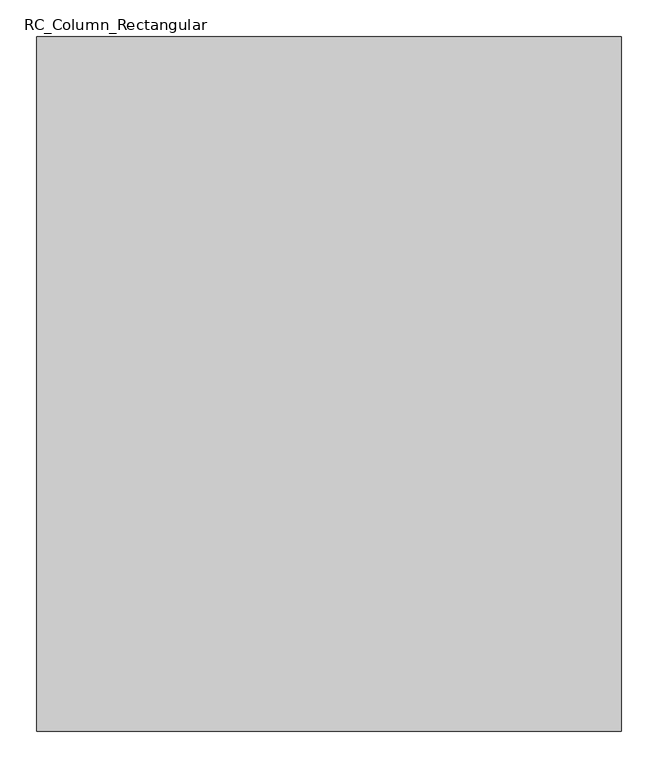
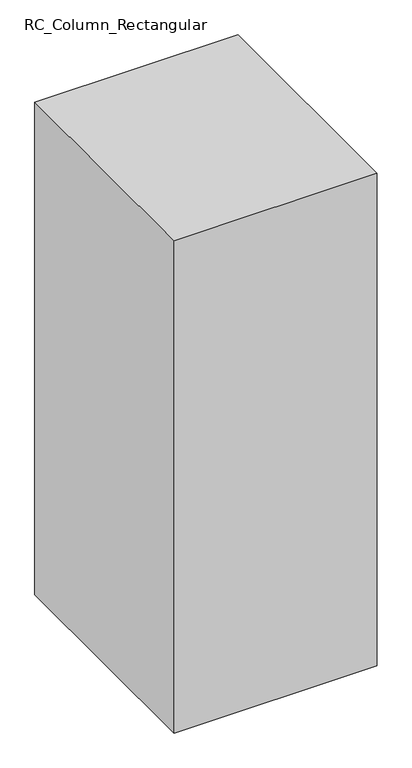
"""IFC4 building model written with IfcOpenShell, lengths in millimetres: column geometry, RC_Column_Rectangular : H_SC_AR_S15_UG PED_W800xL950_Bit_PD1."""

import ifcopenshell
import ifcopenshell.guid

model = None  # the IFC model being written
_history = None  # IfcOwnerHistory: only IFC2X3 demands one
_inside = {}  # id of a spatial element -> (the spatial element, [elements in it])
_under = {}  # id of a project, library or spatial element -> (it, [spatial elements below it])
_declared = {}  # id of a project -> (the project, [libraries it declares])
_typed = {}  # id of a type object -> (the type object, [elements of that type])
_made_of = {}  # id of a material, layer set ... -> (it, [elements and type objects made of it])


def new_model(schema):
    """Start an empty IFC model of exactly this schema.

    Asked for "IFC4X3", IfcOpenShell would pick the latest addendum, in which some entities
    have other attributes; the version numbers below select the first issue.
    IFC2X3 requires an IfcOwnerHistory on every rooted entity: one is made here for all.
    """
    global model, _history
    if schema == "IFC4X3":
        model = ifcopenshell.file(schema_version=(4, 3, 0, 0))
    else:
        model = ifcopenshell.file(schema=schema)
    _inside.clear()
    _under.clear()
    _declared.clear()
    _typed.clear()
    _made_of.clear()
    _history = None
    if model.schema == "IFC2X3":
        org = make("IfcOrganization", Name="unknown")
        user = make(
            "IfcPersonAndOrganization",
            ThePerson=make("IfcPerson", FamilyName="unknown"),
            TheOrganization=org,
        )
        app = make(
            "IfcApplication",
            ApplicationDeveloper=org,
            Version="unknown",
            ApplicationFullName="unknown",
            ApplicationIdentifier="unknown",
        )
        _history = make(
            "IfcOwnerHistory",
            OwningUser=user,
            OwningApplication=app,
            ChangeAction="ADDED",
            CreationDate=0,
        )
    return model


def make(cls, **values):
    """One entity of the class cls with the attributes given. An attribute that is None is left unset."""
    return model.create_entity(
        cls, **{name: value for name, value in values.items() if value is not None}
    )


def rooted(cls, **values):
    """An entity with a GlobalId (a new one), such as an element, a storey or a relation."""
    return make(cls, GlobalId=ifcopenshell.guid.new(), OwnerHistory=_history, **values)


def si_unit(unit_type, name, prefix=None):
    """IfcSIUnit, for example si_unit("LENGTHUNIT", "METRE", prefix="MILLI")."""
    return make("IfcSIUnit", UnitType=unit_type, Prefix=prefix, Name=name)


def assignment(units):
    """IfcUnitAssignment: the units of a project."""
    return None if units is None else make("IfcUnitAssignment", Units=units)


def point(xyz):
    """IfcCartesianPoint."""
    return None if xyz is None else make("IfcCartesianPoint", Coordinates=xyz)


def direction(xyz):
    """IfcDirection."""
    return None if xyz is None else make("IfcDirection", DirectionRatios=xyz)


def frame(location, z_axis=None, x_axis=None):
    """IfcAxis2Placement3D, a coordinate frame: its origin and axes. An axis left out is left unset."""
    return make(
        "IfcAxis2Placement3D",
        Location=point(location),
        Axis=direction(z_axis),
        RefDirection=direction(x_axis),
    )


def origin():
    """The frame at (0, 0, 0) with its axes left unset."""
    return frame((0.0, 0.0, 0.0))


def place(relative_to, where):
    """IfcLocalPlacement: puts the frame where relative to a parent placement (None: the world)."""
    return make(
        "IfcLocalPlacement", PlacementRelTo=relative_to, RelativePlacement=where
    )


def context(
    kind, dimensions, precision=None, world=None, true_north=None, identifier=None
):
    """IfcGeometricRepresentationContext, for example the 3D "Model" context."""
    return make(
        "IfcGeometricRepresentationContext",
        ContextIdentifier=identifier,
        ContextType=kind,
        CoordinateSpaceDimension=dimensions,
        Precision=precision,
        WorldCoordinateSystem=world,
        TrueNorth=true_north,
    )


def project(units=None, contexts=None):
    """IfcProject with its units and contexts."""
    return rooted(
        "IfcProject",
        Name="project",
        RepresentationContexts=contexts,
        UnitsInContext=assignment(units),
    )


def spatial(cls, under=None, at=None, **own):
    """A site, building, storey or space (cls), placed at a placement, below another one or the project."""
    s = rooted(cls, ObjectPlacement=at, **own)
    if under is not None:
        _under.setdefault(under.id(), (under, []))[1].append(s)
    return s


def polyline(points):
    """IfcPolyline through the points."""
    return make("IfcPolyline", Points=[point(p) for p in points])


def outline(outer, holes=None, kind="AREA"):
    """IfcArbitraryClosedProfileDef: a profile drawn as a closed curve; with holes, ...WithVoids."""
    if holes is None:
        return make("IfcArbitraryClosedProfileDef", ProfileType=kind, OuterCurve=outer)
    return make(
        "IfcArbitraryProfileDefWithVoids",
        ProfileType=kind,
        OuterCurve=outer,
        InnerCurves=holes,
    )


def extrude(swept, where, along, depth):
    """IfcExtrudedAreaSolid: the profile swept, set in the frame where, extruded along a direction by depth."""
    return make(
        "IfcExtrudedAreaSolid",
        SweptArea=swept,
        Position=where,
        ExtrudedDirection=direction(along),
        Depth=depth,
    )


def shape(context_of_items, identifier, shape_type, items):
    """IfcShapeRepresentation: the items that make up one representation, for example the "Body"."""
    return make(
        "IfcShapeRepresentation",
        ContextOfItems=context_of_items,
        RepresentationIdentifier=identifier,
        RepresentationType=shape_type,
        Items=items,
    )


def source(mapping_origin, context_of_items, identifier, shape_type, items):
    """IfcRepresentationMap: a shape defined once, which mapped items show again and again."""
    return make(
        "IfcRepresentationMap",
        MappingOrigin=mapping_origin,
        MappedRepresentation=shape(context_of_items, identifier, shape_type, items),
    )


def transform(
    local_origin,
    x_axis=None,
    y_axis=None,
    z_axis=None,
    scale=None,
    scale2=None,
    scale3=None,
    uniform=True,
):
    """IfcCartesianTransformationOperator3D, or its non-uniform kind. x_axis, y_axis, z_axis: its Axis1, 2, 3."""
    if uniform:
        return make(
            "IfcCartesianTransformationOperator3D",
            Axis1=direction(x_axis),
            Axis2=direction(y_axis),
            LocalOrigin=point(local_origin),
            Scale=scale,
            Axis3=direction(z_axis),
        )
    return make(
        "IfcCartesianTransformationOperator3DnonUniform",
        Axis1=direction(x_axis),
        Axis2=direction(y_axis),
        LocalOrigin=point(local_origin),
        Scale=scale,
        Axis3=direction(z_axis),
        Scale2=scale2,
        Scale3=scale3,
    )


def mapped(mapping_source, mapping_target):
    """IfcMappedItem: shows the shape of a source again, moved by a transform."""
    return make(
        "IfcMappedItem", MappingSource=mapping_source, MappingTarget=mapping_target
    )


def made_of(thing, what):
    """Note that an element or type object is made of a material, layer set ...; save() writes the relation."""
    if what is not None:
        _made_of.setdefault(what.id(), (what, []))[1].append(thing)
    return thing


def element(
    cls,
    number,
    at=None,
    inside=None,
    cuts=None,
    type_object=None,
    material=None,
    context=None,
    identifier="Body",
    shape_type=None,
    held_by="IfcProductDefinitionShape",
    body=None,
    shapes=None,
    **own,
):
    """One element of the class cls, such as IfcWall. Its Tag is "e" and its number.

    at: its placement. inside: the storey or other place that contains it. cuts: it is an
    opening in that element (IfcRelVoidsElement). A single representation is given by context,
    identifier, shape_type and body (its items); several are given by shapes. held_by: the class
    of the entity that holds the representations. save() writes the other relations.
    """
    e = rooted(cls, Tag="e%d" % number, ObjectPlacement=at, **own)
    if body is not None:
        shapes = [shape(context, identifier, shape_type, body)]
    if shapes is not None:
        e.Representation = make(held_by, Representations=shapes)
    if inside is not None:
        _inside.setdefault(inside.id(), (inside, []))[1].append(e)
    if cuts is not None:
        rooted(
            "IfcRelVoidsElement", RelatingBuildingElement=cuts, RelatedOpeningElement=e
        )
    if type_object is not None:
        _typed.setdefault(type_object.id(), (type_object, []))[1].append(e)
    return made_of(e, material)


def aggregate(whole, parts):
    """IfcRelAggregates: a whole, such as a stair, and the parts it consists of."""
    return rooted("IfcRelAggregates", RelatingObject=whole, RelatedObjects=parts)


def save(model, path):
    """Write the relations noted so far, then the file.

    IfcRelAggregates (storeys below a building ...), IfcRelContainedInSpatialStructure (elements
    in a storey), IfcRelDefinesByType, IfcRelAssociatesMaterial and IfcRelDeclares: one each for
    every whole, place, type object, material and project.
    """
    for whole, parts in _under.values():
        aggregate(whole, parts)
    for where, things in _inside.values():
        rooted(
            "IfcRelContainedInSpatialStructure",
            RelatedElements=things,
            RelatingStructure=where,
        )
    for kind, things in _typed.values():
        rooted("IfcRelDefinesByType", RelatedObjects=things, RelatingType=kind)
    for what, things in _made_of.values():
        rooted("IfcRelAssociatesMaterial", RelatedObjects=things, RelatingMaterial=what)
    for by, libraries in _declared.values():
        rooted("IfcRelDeclares", RelatingContext=by, RelatedDefinitions=libraries)
    model.write(path)


def rc_column_rectangular_8fcc3407(model_context):
    return source(origin(), model_context, "Body", "SweptSolid", [
        extrude(outline(polyline([(400.0, 475.0), (400.0, -475.0), (-400.0, -475.0), (-400.0, 475.0), (400.0, 475.0)])), frame((0.0, 0.0, -9380.1756499), z_axis=(0.0, 0.0, 1.0), x_axis=(1.0, 0.0, 0.0)), (0.0, 0.0, 1.0), 2050.0),
    ])


if __name__ == "__main__":
    model = new_model("IFC4")
    model_context = context("Model", 3, world=origin())
    ifc_project = project(units=[si_unit("LENGTHUNIT", "METRE", prefix="MILLI")], contexts=[model_context])
    site = spatial("IfcSite", under=ifc_project)
    building = spatial("IfcBuilding", under=site)
    placement = place(None, origin())
    rc_column_rectangular_shape = rc_column_rectangular_8fcc3407(model_context)
    element("IfcColumn", 1, ObjectType="RC_Column_Rectangular : H_SC_AR_S15_UG PED_W800xL950_Bit_PD1", at=placement, inside=building, context=model_context, shape_type="MappedRepresentation", body=[
        mapped(rc_column_rectangular_shape, transform((0.0, 0.0, 0.0), x_axis=(1.0, 0.0, 0.0), y_axis=(0.0, 1.0, 0.0), z_axis=(0.0, 0.0, 1.0))),
    ])
    save(model, "model.ifc")

# Revit data of these elements
# Type "RC_Column_Rectangular : H_SC_AR_S15_UG PED_W800xL950_Bit_PD1"
#   Type Mark = "PD1"
#   Width = 800 mm
#   Length = 950 mm
#   hec_material3 [instance default] = none
#   hec_material2 [instance default] = none
#   hec_material1 [instance default] = none
#   Structural Material [instance default] = none
#   Description = (empty or 0)
